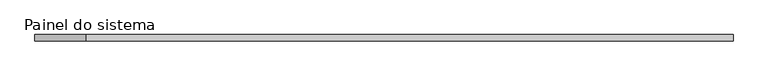
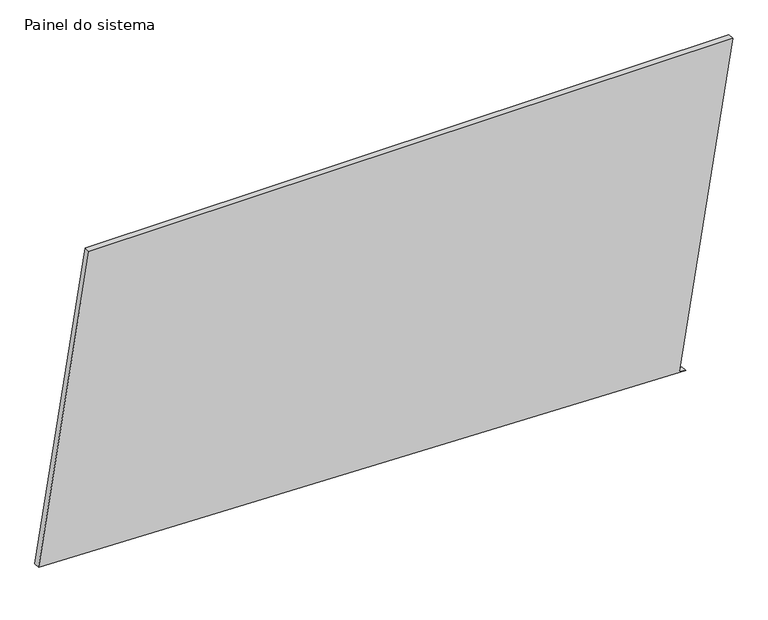
"""IFC4 building model written with IfcOpenShell, lengths in millimetres: plate geometry, Painel do sistema : Envidraçado."""

from ifc_helpers import new_model, si_unit, frame, origin, place, context, project, spatial, polyline, outline, extrude, source, transform, mapped, element, save


def painel_do_sistema_e02cff3a(model_context):
    return source(origin(), model_context, "Body", "SweptSolid", [
        extrude(outline(polyline([(0.0, 1202.4510577), (3.9380954, 1177.7631779), (1340.6739335, 1390.9930405), (1340.6739335, -1188.8447), (73.4080441, -1390.9930405), (0.0, 1202.4510577)])), frame((0.0, 24.5, 0.0), z_axis=(0.0, 1.0, 0.0), x_axis=(0.0, 0.0, 1.0)), (0.0, 0.0, 1.0), 25.0),
    ])


if __name__ == "__main__":
    model = new_model("IFC4")
    model_context = context("Model", 3, world=origin())
    ifc_project = project(units=[si_unit("LENGTHUNIT", "METRE", prefix="MILLI")], contexts=[model_context])
    site = spatial("IfcSite", under=ifc_project)
    building = spatial("IfcBuilding", under=site)
    placement = place(None, origin())
    painel_do_sistema_shape = painel_do_sistema_e02cff3a(model_context)
    element("IfcPlate", 1, ObjectType="Painel do sistema : Envidraçado", at=placement, inside=building, context=model_context, shape_type="MappedRepresentation", body=[
        mapped(painel_do_sistema_shape, transform((0.0, 0.0, 0.0), x_axis=(1.0, 0.0, 0.0), y_axis=(0.0, 1.0, 0.0), z_axis=(0.0, 0.0, 1.0))),
    ])
    save(model, "model.ifc")

# Revit data of these elements
# Type "Painel do sistema : Envidraçado"
#   Construction Type Id = "GSP4R"
#   Analytic Construction = "Vidraça única Pilkington 1/8 pol"
#   Visual Light Transmittance = 0.9
#   Solar Heat Gain Coefficient = 0.86
#   Heat Transfer Coefficient (U) = 6.7069 W/(m²·K)
# Element 1 (IfcPlate, "Painel do sistema : Envidraçado")
#   Materials on its faces: "Vidro"
# Materials
#   "Vidro": class "Vidro", colour RGB 0 128 192, transparency 0.9, Description = "Vidro de sílica", Cost = 0
